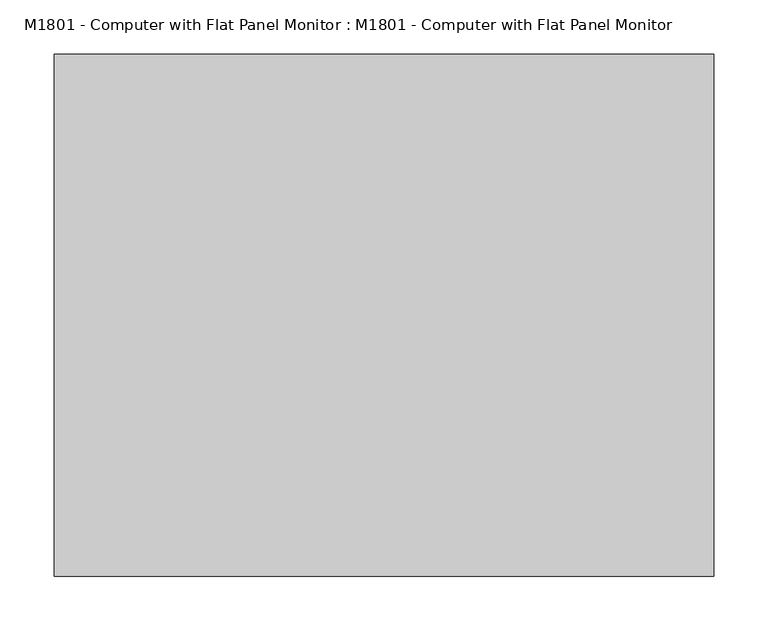
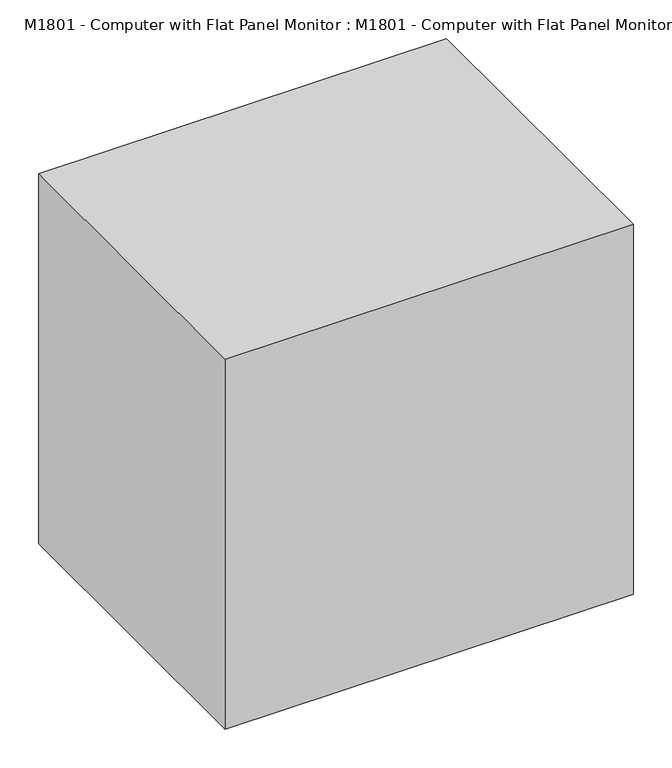
"""IFC4 building model written with IfcOpenShell, lengths in millimetres: proxy geometry, M1801 - Computer with Flat Panel Monitor : M1801 - Computer with Flat Panel Monitor."""

import ifcopenshell
import ifcopenshell.guid

model = None  # the IFC model being written
_history = None  # IfcOwnerHistory: only IFC2X3 demands one
_inside = {}  # id of a spatial element -> (the spatial element, [elements in it])
_under = {}  # id of a project, library or spatial element -> (it, [spatial elements below it])
_declared = {}  # id of a project -> (the project, [libraries it declares])
_typed = {}  # id of a type object -> (the type object, [elements of that type])
_made_of = {}  # id of a material, layer set ... -> (it, [elements and type objects made of it])


def new_model(schema):
    """Start an empty IFC model of exactly this schema.

    Asked for "IFC4X3", IfcOpenShell would pick the latest addendum, in which some entities
    have other attributes; the version numbers below select the first issue.
    IFC2X3 requires an IfcOwnerHistory on every rooted entity: one is made here for all.
    """
    global model, _history
    if schema == "IFC4X3":
        model = ifcopenshell.file(schema_version=(4, 3, 0, 0))
    else:
        model = ifcopenshell.file(schema=schema)
    _inside.clear()
    _under.clear()
    _declared.clear()
    _typed.clear()
    _made_of.clear()
    _history = None
    if model.schema == "IFC2X3":
        org = make("IfcOrganization", Name="unknown")
        user = make(
            "IfcPersonAndOrganization",
            ThePerson=make("IfcPerson", FamilyName="unknown"),
            TheOrganization=org,
        )
        app = make(
            "IfcApplication",
            ApplicationDeveloper=org,
            Version="unknown",
            ApplicationFullName="unknown",
            ApplicationIdentifier="unknown",
        )
        _history = make(
            "IfcOwnerHistory",
            OwningUser=user,
            OwningApplication=app,
            ChangeAction="ADDED",
            CreationDate=0,
        )
    return model


def make(cls, **values):
    """One entity of the class cls with the attributes given. An attribute that is None is left unset."""
    return model.create_entity(
        cls, **{name: value for name, value in values.items() if value is not None}
    )


def rooted(cls, **values):
    """An entity with a GlobalId (a new one), such as an element, a storey or a relation."""
    return make(cls, GlobalId=ifcopenshell.guid.new(), OwnerHistory=_history, **values)


def si_unit(unit_type, name, prefix=None):
    """IfcSIUnit, for example si_unit("LENGTHUNIT", "METRE", prefix="MILLI")."""
    return make("IfcSIUnit", UnitType=unit_type, Prefix=prefix, Name=name)


def assignment(units):
    """IfcUnitAssignment: the units of a project."""
    return None if units is None else make("IfcUnitAssignment", Units=units)


def point(xyz):
    """IfcCartesianPoint."""
    return None if xyz is None else make("IfcCartesianPoint", Coordinates=xyz)


def direction(xyz):
    """IfcDirection."""
    return None if xyz is None else make("IfcDirection", DirectionRatios=xyz)


def frame(location, z_axis=None, x_axis=None):
    """IfcAxis2Placement3D, a coordinate frame: its origin and axes. An axis left out is left unset."""
    return make(
        "IfcAxis2Placement3D",
        Location=point(location),
        Axis=direction(z_axis),
        RefDirection=direction(x_axis),
    )


def origin():
    """The frame at (0, 0, 0) with its axes left unset."""
    return frame((0.0, 0.0, 0.0))


def origin_with_axes():
    """The frame at (0, 0, 0) with the z axis (0, 0, 1) and the x axis (1, 0, 0) written out."""
    return frame((0.0, 0.0, 0.0), z_axis=(0.0, 0.0, 1.0), x_axis=(1.0, 0.0, 0.0))


def place(relative_to, where):
    """IfcLocalPlacement: puts the frame where relative to a parent placement (None: the world)."""
    return make(
        "IfcLocalPlacement", PlacementRelTo=relative_to, RelativePlacement=where
    )


def context(
    kind, dimensions, precision=None, world=None, true_north=None, identifier=None
):
    """IfcGeometricRepresentationContext, for example the 3D "Model" context."""
    return make(
        "IfcGeometricRepresentationContext",
        ContextIdentifier=identifier,
        ContextType=kind,
        CoordinateSpaceDimension=dimensions,
        Precision=precision,
        WorldCoordinateSystem=world,
        TrueNorth=true_north,
    )


def project(units=None, contexts=None):
    """IfcProject with its units and contexts."""
    return rooted(
        "IfcProject",
        Name="project",
        RepresentationContexts=contexts,
        UnitsInContext=assignment(units),
    )


def spatial(cls, under=None, at=None, **own):
    """A site, building, storey or space (cls), placed at a placement, below another one or the project."""
    s = rooted(cls, ObjectPlacement=at, **own)
    if under is not None:
        _under.setdefault(under.id(), (under, []))[1].append(s)
    return s


def polyline(points):
    """IfcPolyline through the points."""
    return make("IfcPolyline", Points=[point(p) for p in points])


def outline(outer, holes=None, kind="AREA"):
    """IfcArbitraryClosedProfileDef: a profile drawn as a closed curve; with holes, ...WithVoids."""
    if holes is None:
        return make("IfcArbitraryClosedProfileDef", ProfileType=kind, OuterCurve=outer)
    return make(
        "IfcArbitraryProfileDefWithVoids",
        ProfileType=kind,
        OuterCurve=outer,
        InnerCurves=holes,
    )


def extrude(swept, where, along, depth):
    """IfcExtrudedAreaSolid: the profile swept, set in the frame where, extruded along a direction by depth."""
    return make(
        "IfcExtrudedAreaSolid",
        SweptArea=swept,
        Position=where,
        ExtrudedDirection=direction(along),
        Depth=depth,
    )


def faces_of(points, faces, orient=None, outer=None):
    """IfcFace entities. A face is a list of loops; a loop is a list of indices into points, from 0.

    orient and outer hold one flag for each loop. By default every Orientation is true, the
    first loop of a face is its IfcFaceOuterBound and the others are IfcFaceBound.
    """
    made = []
    for i, loops in enumerate(faces):
        bounds = []
        for j, loop in enumerate(loops):
            is_outer = j == 0 if outer is None else outer[i][j]
            bounds.append(
                make(
                    "IfcFaceOuterBound" if is_outer else "IfcFaceBound",
                    Bound=make("IfcPolyLoop", Polygon=[points[k] for k in loop]),
                    Orientation=True if orient is None else orient[i][j],
                )
            )
        made.append(make("IfcFace", Bounds=bounds))
    return made


def faceted_brep(points, faces, orient=None, outer=None, voids=None):
    """IfcFacetedBrep: a solid bounded by flat faces; with voids (closed shells), ...WithVoids."""
    shared = [point(p) for p in points]
    hull = make("IfcClosedShell", CfsFaces=faces_of(shared, faces, orient, outer))
    if voids is None:
        return make("IfcFacetedBrep", Outer=hull)
    return make(
        "IfcFacetedBrepWithVoids",
        Outer=hull,
        Voids=[
            make(cls, CfsFaces=faces_of(shared, fs, o, b)) for cls, fs, o, b in voids
        ],
    )


def shape(context_of_items, identifier, shape_type, items):
    """IfcShapeRepresentation: the items that make up one representation, for example the "Body"."""
    return make(
        "IfcShapeRepresentation",
        ContextOfItems=context_of_items,
        RepresentationIdentifier=identifier,
        RepresentationType=shape_type,
        Items=items,
    )


def source(mapping_origin, context_of_items, identifier, shape_type, items):
    """IfcRepresentationMap: a shape defined once, which mapped items show again and again."""
    return make(
        "IfcRepresentationMap",
        MappingOrigin=mapping_origin,
        MappedRepresentation=shape(context_of_items, identifier, shape_type, items),
    )


def transform(
    local_origin,
    x_axis=None,
    y_axis=None,
    z_axis=None,
    scale=None,
    scale2=None,
    scale3=None,
    uniform=True,
):
    """IfcCartesianTransformationOperator3D, or its non-uniform kind. x_axis, y_axis, z_axis: its Axis1, 2, 3."""
    if uniform:
        return make(
            "IfcCartesianTransformationOperator3D",
            Axis1=direction(x_axis),
            Axis2=direction(y_axis),
            LocalOrigin=point(local_origin),
            Scale=scale,
            Axis3=direction(z_axis),
        )
    return make(
        "IfcCartesianTransformationOperator3DnonUniform",
        Axis1=direction(x_axis),
        Axis2=direction(y_axis),
        LocalOrigin=point(local_origin),
        Scale=scale,
        Axis3=direction(z_axis),
        Scale2=scale2,
        Scale3=scale3,
    )


def mapped(mapping_source, mapping_target):
    """IfcMappedItem: shows the shape of a source again, moved by a transform."""
    return make(
        "IfcMappedItem", MappingSource=mapping_source, MappingTarget=mapping_target
    )


def made_of(thing, what):
    """Note that an element or type object is made of a material, layer set ...; save() writes the relation."""
    if what is not None:
        _made_of.setdefault(what.id(), (what, []))[1].append(thing)
    return thing


def element(
    cls,
    number,
    at=None,
    inside=None,
    cuts=None,
    type_object=None,
    material=None,
    context=None,
    identifier="Body",
    shape_type=None,
    held_by="IfcProductDefinitionShape",
    body=None,
    shapes=None,
    **own,
):
    """One element of the class cls, such as IfcWall. Its Tag is "e" and its number.

    at: its placement. inside: the storey or other place that contains it. cuts: it is an
    opening in that element (IfcRelVoidsElement). A single representation is given by context,
    identifier, shape_type and body (its items); several are given by shapes. held_by: the class
    of the entity that holds the representations. save() writes the other relations.
    """
    e = rooted(cls, Tag="e%d" % number, ObjectPlacement=at, **own)
    if body is not None:
        shapes = [shape(context, identifier, shape_type, body)]
    if shapes is not None:
        e.Representation = make(held_by, Representations=shapes)
    if inside is not None:
        _inside.setdefault(inside.id(), (inside, []))[1].append(e)
    if cuts is not None:
        rooted(
            "IfcRelVoidsElement", RelatingBuildingElement=cuts, RelatedOpeningElement=e
        )
    if type_object is not None:
        _typed.setdefault(type_object.id(), (type_object, []))[1].append(e)
    return made_of(e, material)


def aggregate(whole, parts):
    """IfcRelAggregates: a whole, such as a stair, and the parts it consists of."""
    return rooted("IfcRelAggregates", RelatingObject=whole, RelatedObjects=parts)


def save(model, path):
    """Write the relations noted so far, then the file.

    IfcRelAggregates (storeys below a building ...), IfcRelContainedInSpatialStructure (elements
    in a storey), IfcRelDefinesByType, IfcRelAssociatesMaterial and IfcRelDeclares: one each for
    every whole, place, type object, material and project.
    """
    for whole, parts in _under.values():
        aggregate(whole, parts)
    for where, things in _inside.values():
        rooted(
            "IfcRelContainedInSpatialStructure",
            RelatedElements=things,
            RelatingStructure=where,
        )
    for kind, things in _typed.values():
        rooted("IfcRelDefinesByType", RelatedObjects=things, RelatingType=kind)
    for what, things in _made_of.values():
        rooted("IfcRelAssociatesMaterial", RelatedObjects=things, RelatingMaterial=what)
    for by, libraries in _declared.values():
        rooted("IfcRelDeclares", RelatingContext=by, RelatedDefinitions=libraries)
    model.write(path)


def m1801_computer_with_flat_panel_monitor_m1801_computer_with_cf90e1c8(model_context):
    return source(origin(), model_context, "Body", "SolidModel", [
        faceted_brep([(203.2, 133.2656905, 431.8), (-203.2, 133.2656905, 431.8), (-203.2, 82.6343095, 431.8), (203.2, 82.6343095, 431.8), (203.2, 133.2656905, 152.4), (203.2, 82.6343095, 152.4), (-203.2, 82.6343095, 152.4), (-203.2, 133.2656905, 152.4), (-190.5, 82.6343095, 419.1), (190.5, 82.6343095, 419.1), (190.5, 82.6343095, 165.1), (-190.5, 82.6343095, 165.1), (190.5, 87.4205119, 419.1), (-190.5, 87.4205119, 419.1), (190.5, 87.4205119, 165.1), (-190.5, 87.4205119, 165.1)], [[[0, 1, 2, 3]], [[4, 5, 6, 7]], [[1, 0, 4, 7]], [[2, 1, 7, 6]], [[3, 2, 6, 5], [8, 9, 10, 11]], [[0, 3, 5, 4]], [[12, 9, 8, 13]], [[14, 15, 11, 10]], [[12, 13, 15, 14]], [[13, 8, 11, 15]], [[9, 12, 14, 10]]]),
        faceted_brep([(109.1218395, 34.0676261, 25.4), (109.1218395, 34.0676261, 0.0), (109.1218395, 215.9, 0.0), (109.1218395, 215.9, 25.4), (-109.1218395, 215.9, 25.4), (-109.1218395, 215.9, 0.0), (-109.1218395, 34.0676261, 0.0), (-109.1218395, 34.0676261, 25.4), (36.9685686, 196.7656905, 31.75), (36.9685686, 196.7656905, 25.4), (-36.9685686, 196.7656905, 25.4), (-36.9685686, 196.7656905, 31.75), (36.9685686, 196.7656905, 292.1), (-36.9685686, 196.7656905, 292.1), (36.9685686, 133.2656905, 292.1), (-36.9685686, 133.2656905, 292.1), (36.9685686, 133.2656905, 241.3), (-36.9685686, 133.2656905, 241.3), (36.9685686, 171.3656905, 241.3), (-36.9685686, 171.3656905, 241.3), (36.9685686, 171.3656905, 25.4), (-36.9685686, 171.3656905, 25.4)], [[[0, 1, 2, 3]], [[4, 5, 6, 7]], [[8, 9, 10, 11]], [[12, 8, 11, 13]], [[14, 12, 13, 15]], [[16, 14, 15, 17]], [[18, 16, 17, 19]], [[20, 18, 19, 21]], [[0, 3, 4, 7], [9, 20, 21, 10]], [[1, 0, 7, 6]], [[2, 1, 6, 5]], [[3, 2, 5, 4]], [[20, 9, 8, 12, 14, 16, 18]], [[10, 21, 19, 17, 15, 13, 11]]]),
        extrude(outline(polyline([(-171.45, 0.0), (-171.45, 12.7), (-19.05, 25.4), (-19.05, 0.0), (-171.45, 0.0)])), frame((-203.2, 0.0, 0.0), z_axis=(1.0, 0.0, 0.0), x_axis=(0.0, 1.0, 0.0)), (0.0, 0.0, 1.0), 406.4),
        extrude(outline(polyline([(304.8, 241.3), (304.8, -241.3), (-304.8, -241.3), (-304.8, 241.3), (304.8, 241.3)])), origin_with_axes(), (0.0, 0.0, 1.0), 584.2),
    ])


if __name__ == "__main__":
    model = new_model("IFC4")
    model_context = context("Model", 3, world=origin())
    ifc_project = project(units=[si_unit("LENGTHUNIT", "METRE", prefix="MILLI")], contexts=[model_context])
    site = spatial("IfcSite", under=ifc_project)
    building = spatial("IfcBuilding", under=site)
    placement = place(None, origin())
    m1801_computer_with_flat_panel_monitor_m1801_computer_with_shape = m1801_computer_with_flat_panel_monitor_m1801_computer_with_cf90e1c8(model_context)
    element("IfcBuildingElementProxy", 1, Name="M1801 - Computer with Flat Panel Monitor : M1801 - Computer with Flat Panel Monitor", ObjectType="M1801 - Computer with Flat Panel Monitor : M1801 - Computer with Flat Panel Monitor", at=placement, inside=building, context=model_context, shape_type="MappedRepresentation", body=[
        mapped(m1801_computer_with_flat_panel_monitor_m1801_computer_with_shape, transform((0.0, 0.0, 0.0), x_axis=(1.0, 0.0, 0.0), y_axis=(0.0, 1.0, 0.0), z_axis=(0.0, 0.0, 1.0))),
    ])
    save(model, "model.ifc")

# Revit data of these elements
# Type "M1801 - Computer with Flat Panel Monitor : M1801 - Computer with Flat Panel Monitor"
#   Watts2 = "0"
#   Watts1 = "600"
#   Unit_Issue = "EA"
#   UTIL_6_Misc = "-"
#   UTIL_5_NonMedGas = "-"
#   UTIL_4_MiscGas = "-"
#   UTIL_3_MedGas = "-"
#   UTIL_2_Elec = "A"
#   UTIL_1_WaterDrain = "-"
#   Nomenclature = "Computer, Microprocessing, w/Flat Panel Monitor"
#   NSN = "7025"
#   Location [instance default] = ""
#   JSN = "M1801"
#   Fund_Source_VA = "-"
#   Fund_Source_Navy = "-"
#   Fund_Source_Army = "-"
#   Fund_Source_AF = "-"
#   ELEC_Volts2 = "0"
#   ELEC_Volts1 = "120"
#   ELEC_Phase2 = "0"
#   ELEC_Phase1 = "1"
#   ELEC_HertzSwitch = "1"
#   ELEC_HertzDependent = "0"
#   ELEC_Hertz = "60"
#   ELEC_Amps2 = "0"
#   ELEC_Amps1 = "5"
#   DetailDescription = "Desk top microprocessing computer. The unit shall consist of a central processing mini tower, flat panel monitor, keyboard, mouse and speakers. The system shall have the following minimum characteristics: a 2.8 GHz Pentium processor; 512 MB memory; 80GB hard drive; 32/48x CD-ROMDVD combo; 1.44MB network interface card; video 32 MB NVIDIA; a 18 inch flat panel monitor. The computer is used throughout the facility to input, manipulate and retrieve information."
#   CAT_VA = "C"
#   CAT_Navy = "C"
#   CAT_IHS = "-"
#   CAT_Army = "C"
#   CAT_AF = "C"
#   BTUperhour = "0"
#   Weight_IP = 45
#   DIM_Width_IP = 2' - 0"
#   DIM_Height_IP = 1' - 11"
#   DIM_Depth_IP = 1' - 7"
#   Assembly Code = ""
# Element 1 (IfcBuildingElementProxy, "M1801 - Computer with Flat Panel Monitor : M1801 - Computer with Flat Panel Monitor")
#   Materials on its faces: "EquipSpace"
# Materials
#   "EquipSpace": class "Unassigned", colour RGB 221 217 195, transparency 0.5
